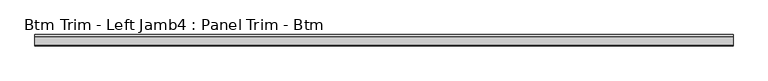
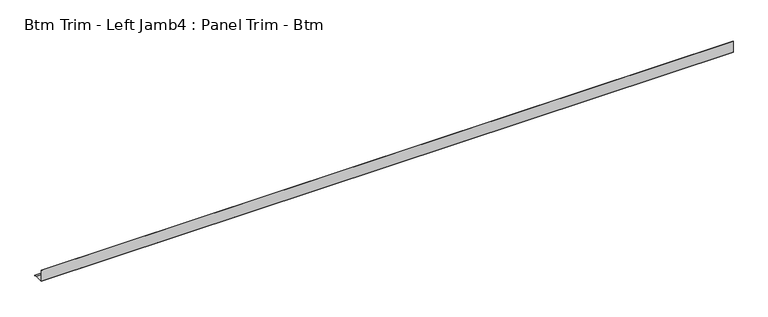
"""IFC4 building model written with IfcOpenShell, lengths in millimetres: proxy geometry, Btm Trim - Left Jamb4 : Panel Trim - Btm."""

from ifc_helpers import new_model, si_unit, frame, origin, place, context, project, spatial, polyline, outline, extrude, source, transform, mapped, element, save


def btm_trim_left_jamb4_panel_trim_btm_b9c60ca2(model_context):
    return source(origin(), model_context, "Body", "SweptSolid", [
        extrude(outline(polyline([(-531600.2244849, 0.79375), (-531590.923103, -1.6985478), (-531591.1285406, -2.4652514), (-531600.3289841, 0.0), (-531640.0037841, 0.0), (-531640.0037841, 51.59375), (-531639.2163841, 51.59375), (-531639.2163841, 0.79375), (-531600.2244849, 0.79375)])), frame((587327.7998239, 0.0, 0.0), z_axis=(1.0, 0.0, 0.0), x_axis=(0.0, 1.0, 0.0)), (0.0, 0.0, 1.0), 3063.2733375),
    ])


if __name__ == "__main__":
    model = new_model("IFC4")
    model_context = context("Model", 3, world=origin())
    ifc_project = project(units=[si_unit("LENGTHUNIT", "METRE", prefix="MILLI")], contexts=[model_context])
    site = spatial("IfcSite", under=ifc_project)
    building = spatial("IfcBuilding", under=site)
    placement = place(None, origin())
    btm_trim_left_jamb4_panel_trim_btm_shape = btm_trim_left_jamb4_panel_trim_btm_b9c60ca2(model_context)
    element("IfcBuildingElementProxy", 1, Name="Btm Trim - Left Jamb4 : Panel Trim - Btm", ObjectType="Btm Trim - Left Jamb4 : Panel Trim - Btm", at=placement, inside=building, context=model_context, shape_type="MappedRepresentation", body=[
        mapped(btm_trim_left_jamb4_panel_trim_btm_shape, transform((0.0, 0.0, 0.0), x_axis=(1.0, 0.0, 0.0), y_axis=(0.0, 1.0, 0.0), z_axis=(0.0, 0.0, 1.0))),
    ])
    save(model, "model.ifc")

# Revit data of these elements
# Element 1 (IfcBuildingElementProxy, "Btm Trim - Left Jamb4 : Panel Trim - Btm")
#   Materials on its faces: "BASE TRIM BY MTL PANEL MFR."
# Materials
#   "BASE TRIM BY MTL PANEL MFR.": class "Generic", colour RGB 239 242 240, transparency 0, Cost = 0
